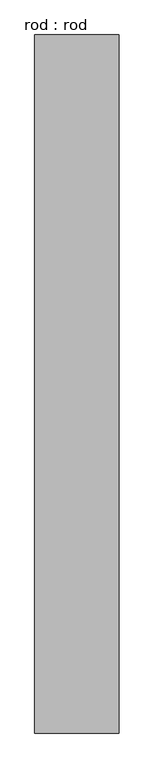
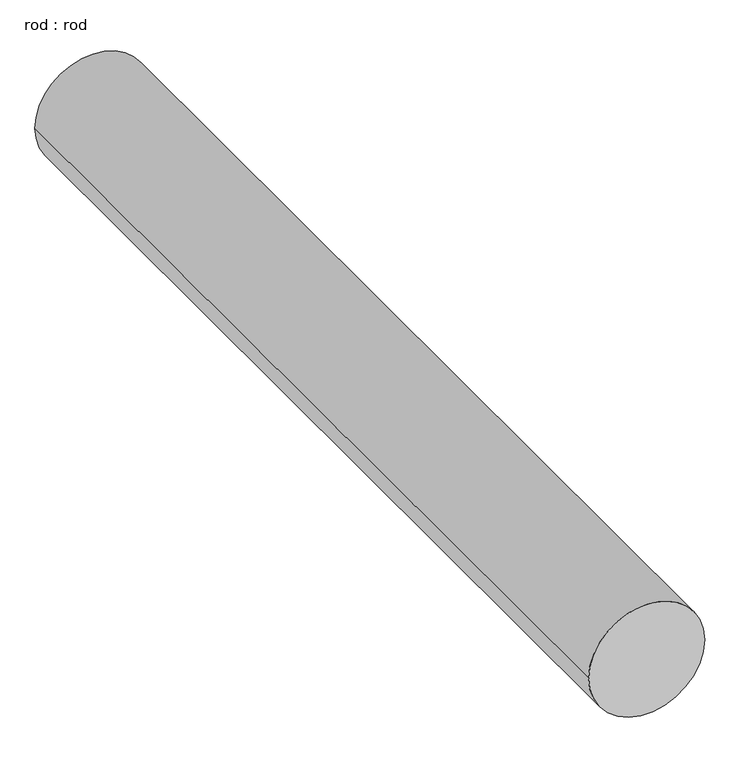
"""IFC4 building model written with IfcOpenShell, lengths in millimetres: proxy geometry, rod : rod."""

from ifc_helpers import new_model, si_unit, point, frame, frame_2d, origin, place, context, project, spatial, circle_curve, trimmed, segment, composite_curve, outline, extrude, source, transform, mapped, element, save


def rod_rod_6cdf31df(model_context):
    return source(origin(), model_context, "Body", "SweptSolid", [
        extrude(outline(composite_curve([segment(trimmed(circle_curve(frame_2d((0.0108462, 0.0)), 200.0), [point((0.0108462, 200.0))], [point((0.0108462, -200.0))], False, "CARTESIAN"), True, "CONTINUOUS"), segment(trimmed(circle_curve(frame_2d((0.0108462, 0.0)), 200.0), [point((0.0108462, -200.0))], [point((0.0108462, 200.0))], False, "CARTESIAN"), True, "CONTINUOUS")], self_intersect=False)), frame((0.0, 2437.3714725, 0.0), z_axis=(0.0, 1.0, 0.0), x_axis=(0.0, 0.0, 1.0)), (0.0, 0.0, 1.0), 3310.7142857),
    ])


if __name__ == "__main__":
    model = new_model("IFC4")
    model_context = context("Model", 3, world=origin())
    ifc_project = project(units=[si_unit("LENGTHUNIT", "METRE", prefix="MILLI")], contexts=[model_context])
    site = spatial("IfcSite", under=ifc_project)
    building = spatial("IfcBuilding", under=site)
    placement = place(None, origin())
    rod_rod_shape = rod_rod_6cdf31df(model_context)
    element("IfcBuildingElementProxy", 1, Name="rod : rod", ObjectType="rod : rod", at=placement, inside=building, context=model_context, shape_type="MappedRepresentation", body=[
        mapped(rod_rod_shape, transform((0.0, 0.0, 0.0), x_axis=(1.0, 0.0, 0.0), y_axis=(0.0, 1.0, 0.0), z_axis=(0.0, 0.0, 1.0))),
    ])
    save(model, "model.ifc")

# Revit data of these elements
# Type "rod : rod"
#   Default Elevation = 0
